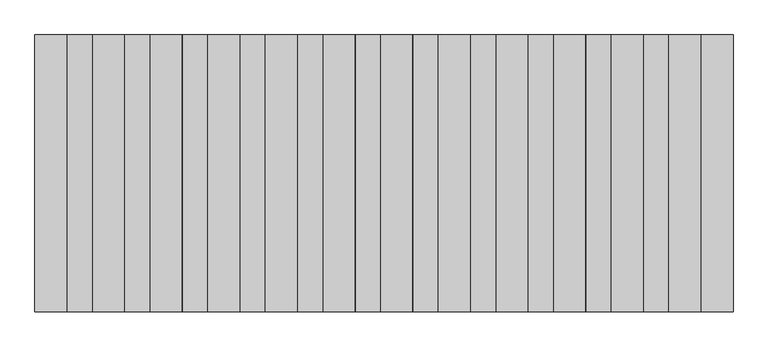
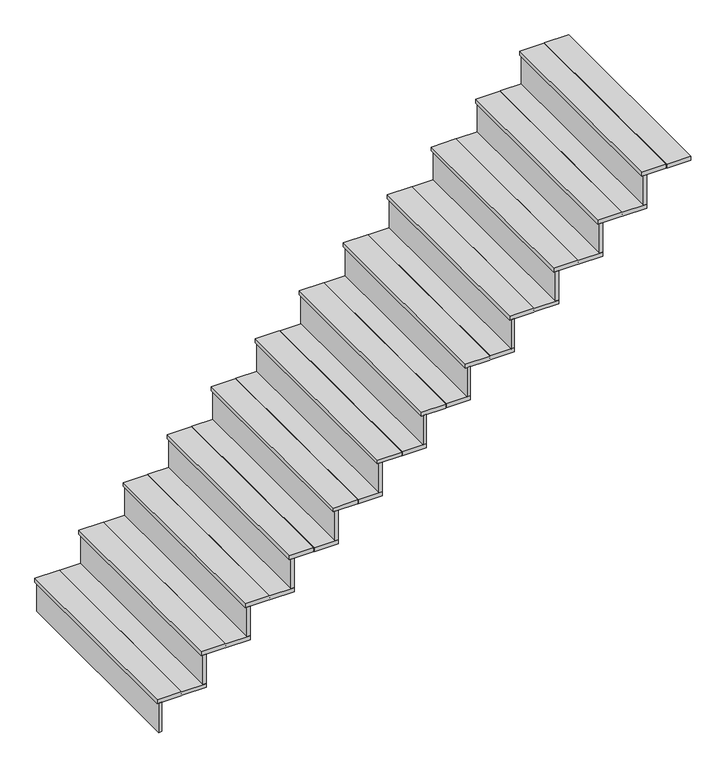
"""IFC4 building model written with IfcOpenShell, lengths in millimetres: stair flight geometry."""

from ifc_helpers import new_model, si_unit, frame, origin, place, context, project, spatial, polyline, outline, extrude, source, transform, mapped, element, save


def stair_flight_14335fb9(model_context):
    return source(origin(), model_context, "Body", "SweptSolid", [
        extrude(outline(polyline([(34837.3896626, 5952.9710177), (34818.3396626, 5952.9710177), (34818.3396626, 7172.1710177), (34837.3896626, 7172.1710177), (34837.3896626, 5952.9710177)])), frame((0.0, 0.0, -2438.4), z_axis=(0.0, 0.0, 1.0), x_axis=(1.0, 0.0, 0.0)), (0.0, 0.0, 1.0), 179.2882813),
        extrude(outline(polyline([(-2259.1117187, 34948.5146626), (-2247.3574467, 34948.5146626), (-2247.3574467, 34951.6896626), (-2259.1117188, 34951.6896626), (-2259.1117188, 35091.3896626), (-2235.2, 35091.3896626), (-2235.2, 34951.6896626), (-2246.9542721, 34951.6896626), (-2246.9542721, 34948.5146626), (-2235.2, 34948.5146626), (-2235.2, 34808.8146626), (-2259.1117187, 34808.8146626), (-2259.1117187, 34948.5146626)])), frame((0.0, 5952.9710177, 0.0), z_axis=(0.0, 1.0, 0.0), x_axis=(0.0, 0.0, 1.0)), (0.0, 0.0, 1.0), 1219.2),
        extrude(outline(polyline([(35091.3896626, 5952.9710177), (35072.3396626, 5952.9710177), (35072.3396626, 7172.1710177), (35091.3896626, 7172.1710177), (35091.3896626, 5952.9710177)])), frame((0.0, 0.0, -2235.2), z_axis=(0.0, 0.0, 1.0), x_axis=(1.0, 0.0, 0.0)), (0.0, 0.0, 1.0), 179.2882813),
        extrude(outline(polyline([(-2055.9117188, 35202.5146626), (-2044.1574467, 35202.5146626), (-2044.1574467, 35205.6896626), (-2055.9117188, 35205.6896626), (-2055.9117188, 35345.3896626), (-2032.0, 35345.3896626), (-2032.0, 35205.6896626), (-2043.7542721, 35205.6896626), (-2043.7542721, 35202.5146626), (-2032.0, 35202.5146626), (-2032.0, 35062.8146626), (-2055.9117188, 35062.8146626), (-2055.9117188, 35202.5146626)])), frame((0.0, 5952.9710177, 0.0), z_axis=(0.0, 1.0, 0.0), x_axis=(0.0, 0.0, 1.0)), (0.0, 0.0, 1.0), 1219.2),
        extrude(outline(polyline([(35345.3896626, 5952.9710177), (35326.3396626, 5952.9710177), (35326.3396626, 7172.1710177), (35345.3896626, 7172.1710177), (35345.3896626, 5952.9710177)])), frame((0.0, 0.0, -2032.0), z_axis=(0.0, 0.0, 1.0), x_axis=(1.0, 0.0, 0.0)), (0.0, 0.0, 1.0), 179.2882813),
        extrude(outline(polyline([(-1852.7117188, 35456.5146626), (-1840.9574467, 35456.5146626), (-1840.9574467, 35459.6896626), (-1852.7117188, 35459.6896626), (-1852.7117188, 35599.3896626), (-1828.8, 35599.3896626), (-1828.8, 35459.6896626), (-1840.5542721, 35459.6896626), (-1840.5542721, 35456.5146626), (-1828.8, 35456.5146626), (-1828.8, 35316.8146626), (-1852.7117188, 35316.8146626), (-1852.7117188, 35456.5146626)])), frame((0.0, 5952.9710177, 0.0), z_axis=(0.0, 1.0, 0.0), x_axis=(0.0, 0.0, 1.0)), (0.0, 0.0, 1.0), 1219.2),
        extrude(outline(polyline([(35599.3896626, 5952.9710177), (35580.3396626, 5952.9710177), (35580.3396626, 7172.1710177), (35599.3896626, 7172.1710177), (35599.3896626, 5952.9710177)])), frame((0.0, 0.0, -1828.8), z_axis=(0.0, 0.0, 1.0), x_axis=(1.0, 0.0, 0.0)), (0.0, 0.0, 1.0), 179.2882813),
        extrude(outline(polyline([(-1649.5117188, 35710.5146626), (-1637.7574467, 35710.5146626), (-1637.7574467, 35713.6896626), (-1649.5117188, 35713.6896626), (-1649.5117188, 35853.3896626), (-1625.6, 35853.3896626), (-1625.6, 35713.6896626), (-1637.3542721, 35713.6896626), (-1637.3542721, 35710.5146626), (-1625.6, 35710.5146626), (-1625.6, 35570.8146626), (-1649.5117188, 35570.8146626), (-1649.5117188, 35710.5146626)])), frame((0.0, 5952.9710177, 0.0), z_axis=(0.0, 1.0, 0.0), x_axis=(0.0, 0.0, 1.0)), (0.0, 0.0, 1.0), 1219.2),
        extrude(outline(polyline([(35853.3896626, 5952.9710177), (35834.3396626, 5952.9710177), (35834.3396626, 7172.1710177), (35853.3896626, 7172.1710177), (35853.3896626, 5952.9710177)])), frame((0.0, 0.0, -1625.6), z_axis=(0.0, 0.0, 1.0), x_axis=(1.0, 0.0, 0.0)), (0.0, 0.0, 1.0), 179.2882813),
        extrude(outline(polyline([(-1446.3117187, 35964.5146626), (-1434.5574467, 35964.5146626), (-1434.5574467, 35967.6896626), (-1446.3117188, 35967.6896626), (-1446.3117188, 36107.3896626), (-1422.4, 36107.3896626), (-1422.4, 35967.6896626), (-1434.1542721, 35967.6896626), (-1434.1542721, 35964.5146626), (-1422.4, 35964.5146626), (-1422.4, 35824.8146626), (-1446.3117187, 35824.8146626), (-1446.3117187, 35964.5146626)])), frame((0.0, 5952.9710177, 0.0), z_axis=(0.0, 1.0, 0.0), x_axis=(0.0, 0.0, 1.0)), (0.0, 0.0, 1.0), 1219.2),
        extrude(outline(polyline([(36107.3896626, 5952.9710177), (36088.3396626, 5952.9710177), (36088.3396626, 7172.1710177), (36107.3896626, 7172.1710177), (36107.3896626, 5952.9710177)])), frame((0.0, 0.0, -1422.4), z_axis=(0.0, 0.0, 1.0), x_axis=(1.0, 0.0, 0.0)), (0.0, 0.0, 1.0), 179.2882813),
        extrude(outline(polyline([(-1243.1117187, 36218.5146626), (-1231.3574467, 36218.5146626), (-1231.3574467, 36221.6896626), (-1243.1117188, 36221.6896626), (-1243.1117188, 36361.3896626), (-1219.2, 36361.3896626), (-1219.2, 36221.6896626), (-1230.9542721, 36221.6896626), (-1230.9542721, 36218.5146626), (-1219.2, 36218.5146626), (-1219.2, 36078.8146626), (-1243.1117187, 36078.8146626), (-1243.1117187, 36218.5146626)])), frame((0.0, 5952.9710177, 0.0), z_axis=(0.0, 1.0, 0.0), x_axis=(0.0, 0.0, 1.0)), (0.0, 0.0, 1.0), 1219.2),
        extrude(outline(polyline([(36361.3896626, 5952.9710177), (36342.3396626, 5952.9710177), (36342.3396626, 7172.1710177), (36361.3896626, 7172.1710177), (36361.3896626, 5952.9710177)])), frame((0.0, 0.0, -1219.2), z_axis=(0.0, 0.0, 1.0), x_axis=(1.0, 0.0, 0.0)), (0.0, 0.0, 1.0), 179.2882813),
        extrude(outline(polyline([(-1039.9117188, 36472.5146626), (-1028.1574467, 36472.5146626), (-1028.1574467, 36475.6896626), (-1039.9117188, 36475.6896626), (-1039.9117188, 36615.3896626), (-1016.0, 36615.3896626), (-1016.0, 36475.6896626), (-1027.7542721, 36475.6896626), (-1027.7542721, 36472.5146626), (-1016.0, 36472.5146626), (-1016.0, 36332.8146626), (-1039.9117188, 36332.8146626), (-1039.9117188, 36472.5146626)])), frame((0.0, 5952.9710177, 0.0), z_axis=(0.0, 1.0, 0.0), x_axis=(0.0, 0.0, 1.0)), (0.0, 0.0, 1.0), 1219.2),
        extrude(outline(polyline([(36615.3896626, 5952.9710177), (36596.3396626, 5952.9710177), (36596.3396626, 7172.1710177), (36615.3896626, 7172.1710177), (36615.3896626, 5952.9710177)])), frame((0.0, 0.0, -1016.0), z_axis=(0.0, 0.0, 1.0), x_axis=(1.0, 0.0, 0.0)), (0.0, 0.0, 1.0), 179.2882813),
        extrude(outline(polyline([(-836.7117188, 36726.5146626), (-824.9574467, 36726.5146626), (-824.9574467, 36729.6896626), (-836.7117188, 36729.6896626), (-836.7117188, 36869.3896626), (-812.8, 36869.3896626), (-812.8, 36729.6896626), (-824.5542721, 36729.6896626), (-824.5542721, 36726.5146626), (-812.8, 36726.5146626), (-812.8, 36586.8146626), (-836.7117188, 36586.8146626), (-836.7117188, 36726.5146626)])), frame((0.0, 5952.9710177, 0.0), z_axis=(0.0, 1.0, 0.0), x_axis=(0.0, 0.0, 1.0)), (0.0, 0.0, 1.0), 1219.2),
        extrude(outline(polyline([(36869.3896626, 5952.9710177), (36850.3396626, 5952.9710177), (36850.3396626, 7172.1710177), (36869.3896626, 7172.1710177), (36869.3896626, 5952.9710177)])), frame((0.0, 0.0, -812.8), z_axis=(0.0, 0.0, 1.0), x_axis=(1.0, 0.0, 0.0)), (0.0, 0.0, 1.0), 179.2882813),
        extrude(outline(polyline([(-633.5117188, 36980.5146626), (-621.7574467, 36980.5146626), (-621.7574467, 36983.6896626), (-633.5117188, 36983.6896626), (-633.5117188, 37123.3896626), (-609.6, 37123.3896626), (-609.6, 36983.6896626), (-621.3542721, 36983.6896626), (-621.3542721, 36980.5146626), (-609.6, 36980.5146626), (-609.6, 36840.8146626), (-633.5117188, 36840.8146626), (-633.5117188, 36980.5146626)])), frame((0.0, 5952.9710177, 0.0), z_axis=(0.0, 1.0, 0.0), x_axis=(0.0, 0.0, 1.0)), (0.0, 0.0, 1.0), 1219.2),
        extrude(outline(polyline([(37123.3896626, 5952.9710177), (37104.3396626, 5952.9710177), (37104.3396626, 7172.1710177), (37123.3896626, 7172.1710177), (37123.3896626, 5952.9710177)])), frame((0.0, 0.0, -609.6), z_axis=(0.0, 0.0, 1.0), x_axis=(1.0, 0.0, 0.0)), (0.0, 0.0, 1.0), 179.2882813),
        extrude(outline(polyline([(-430.3117188, 37234.5146626), (-418.5574467, 37234.5146626), (-418.5574467, 37237.6896626), (-430.3117188, 37237.6896626), (-430.3117188, 37377.3896626), (-406.4, 37377.3896626), (-406.4, 37237.6896626), (-418.1542721, 37237.6896626), (-418.1542721, 37234.5146626), (-406.4, 37234.5146626), (-406.4, 37094.8146626), (-430.3117188, 37094.8146626), (-430.3117188, 37234.5146626)])), frame((0.0, 5952.9710177, 0.0), z_axis=(0.0, 1.0, 0.0), x_axis=(0.0, 0.0, 1.0)), (0.0, 0.0, 1.0), 1219.2),
        extrude(outline(polyline([(37377.3896626, 5952.9710177), (37358.3396626, 5952.9710177), (37358.3396626, 7172.1710177), (37377.3896626, 7172.1710177), (37377.3896626, 5952.9710177)])), frame((0.0, 0.0, -406.4), z_axis=(0.0, 0.0, 1.0), x_axis=(1.0, 0.0, 0.0)), (0.0, 0.0, 1.0), 179.2882813),
        extrude(outline(polyline([(-227.1117187, 37488.5146626), (-215.3574467, 37488.5146626), (-215.3574467, 37491.6896626), (-227.1117188, 37491.6896626), (-227.1117188, 37631.3896626), (-203.2, 37631.3896626), (-203.2, 37491.6896626), (-214.9542721, 37491.6896626), (-214.9542721, 37488.5146626), (-203.2, 37488.5146626), (-203.2, 37348.8146626), (-227.1117187, 37348.8146626), (-227.1117187, 37488.5146626)])), frame((0.0, 5952.9710177, 0.0), z_axis=(0.0, 1.0, 0.0), x_axis=(0.0, 0.0, 1.0)), (0.0, 0.0, 1.0), 1219.2),
        extrude(outline(polyline([(37631.3896626, 5952.9710177), (37612.3396626, 5952.9710177), (37612.3396626, 7172.1710177), (37631.3896626, 7172.1710177), (37631.3896626, 5952.9710177)])), frame((0.0, 0.0, -203.2), z_axis=(0.0, 0.0, 1.0), x_axis=(1.0, 0.0, 0.0)), (0.0, 0.0, 1.0), 179.2882812),
        extrude(outline(polyline([(-23.9117188, 37742.5146626), (-12.1574467, 37742.5146626), (-12.1574467, 37745.6896626), (-23.9117188, 37745.6896626), (-23.9117188, 37885.3896626), (0.0, 37885.3896626), (0.0, 37745.6896626), (-11.7542721, 37745.6896626), (-11.7542721, 37742.5146626), (0.0, 37742.5146626), (0.0, 37602.8146626), (-23.9117188, 37602.8146626), (-23.9117188, 37742.5146626)])), frame((0.0, 5952.9710177, 0.0), z_axis=(0.0, 1.0, 0.0), x_axis=(0.0, 0.0, 1.0)), (0.0, 0.0, 1.0), 1219.2),
    ])


if __name__ == "__main__":
    model = new_model("IFC4")
    model_context = context("Model", 3, world=origin())
    ifc_project = project(units=[si_unit("LENGTHUNIT", "METRE", prefix="MILLI")], contexts=[model_context])
    site = spatial("IfcSite", under=ifc_project)
    building = spatial("IfcBuilding", under=site)
    placement = place(None, origin())
    stair_flight_shape = stair_flight_14335fb9(model_context)
    element("IfcStairFlight", 1, at=placement, inside=building, context=model_context, shape_type="MappedRepresentation", body=[
        mapped(stair_flight_shape, transform((0.0, 0.0, 0.0), x_axis=(1.0, 0.0, 0.0), y_axis=(0.0, 1.0, 0.0), z_axis=(0.0, 0.0, 1.0))),
    ])
    save(model, "model.ifc")

# Revit data of these elements
# Element 1 (IfcStairFlight)
#   Materials on its faces: "COMPOSITE DECKING"
# Materials
#   "COMPOSITE DECKING": class "Wood", colour RGB 120 75 45, transparency 0, Keynote = "06 11 00", Model = "Trex Select® Composite Deck 1\" Grooved Edge Board", Manufacturer = "Trex", URL = "http://www.trex.com/", Description = "1x6 Trex Select® Composite Deck Grooved Edge Board", Cost = 0
